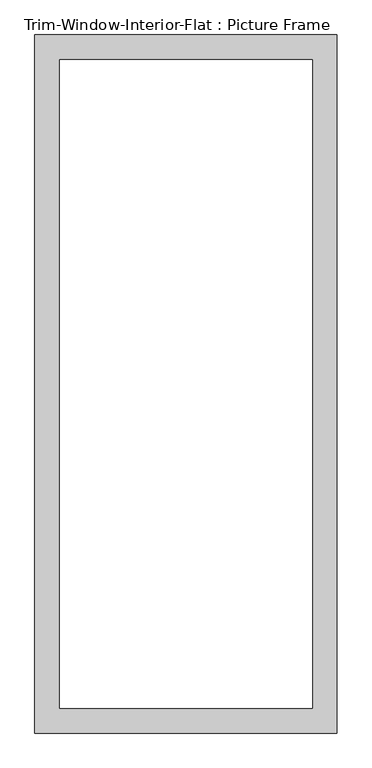
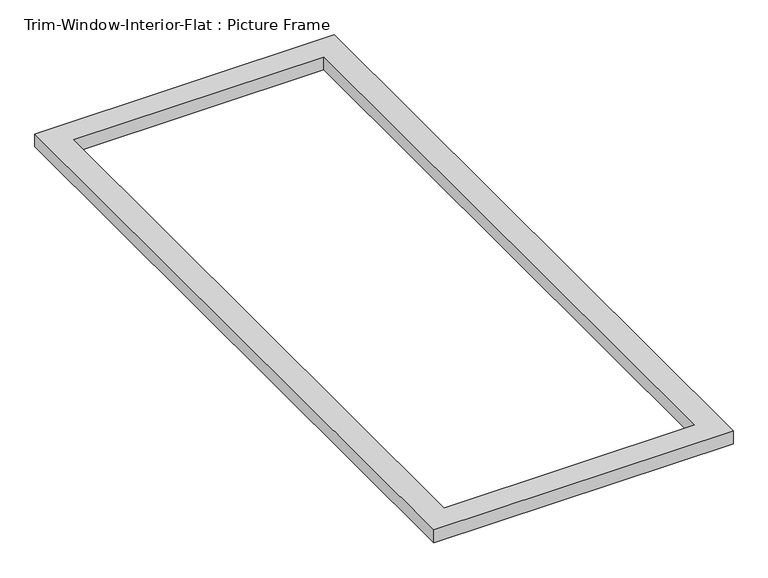
"""IFC4 building model written with IfcOpenShell, lengths in millimetres: proxy geometry, Trim-Window-Interior-Flat : Picture Frame."""

from ifc_helpers import new_model, si_unit, origin, origin_with_axes, place, context, project, spatial, polyline, outline, extrude, source, transform, mapped, element, save


def trim_window_interior_flat_picture_frame_70b72581(model_context):
    return source(origin(), model_context, "Body", "SweptSolid", [
        extrude(outline(polyline([(349.25, -44.45), (-349.25, -44.45), (-349.25, 1568.45), (349.25, 1568.45), (349.25, -44.45)]), holes=[polyline([(292.1, 12.7), (292.1, 1511.3), (-292.1, 1511.3), (-292.1, 12.7), (292.1, 12.7)])]), origin_with_axes(), (0.0, 0.0, 1.0), 31.75),
    ])


if __name__ == "__main__":
    model = new_model("IFC4")
    model_context = context("Model", 3, world=origin())
    ifc_project = project(units=[si_unit("LENGTHUNIT", "METRE", prefix="MILLI")], contexts=[model_context])
    site = spatial("IfcSite", under=ifc_project)
    building = spatial("IfcBuilding", under=site)
    placement = place(None, origin())
    trim_window_interior_flat_picture_frame_shape = trim_window_interior_flat_picture_frame_70b72581(model_context)
    element("IfcBuildingElementProxy", 1, Name="Trim-Window-Interior-Flat : Picture Frame", ObjectType="Trim-Window-Interior-Flat : Picture Frame", at=placement, inside=building, context=model_context, shape_type="MappedRepresentation", body=[
        mapped(trim_window_interior_flat_picture_frame_shape, transform((0.0, 0.0, 0.0), x_axis=(1.0, 0.0, 0.0), y_axis=(0.0, 1.0, 0.0), z_axis=(0.0, 0.0, 1.0))),
    ])
    save(model, "model.ifc")

# Revit data of these elements
# Type "Trim-Window-Interior-Flat : Picture Frame"
#   Trim Thickness_Picture Frame = 0' - 1 1/4"
#   Trim Width = 0' - 2 1/4"
#   Trim Thickness_with Sill = 0' - 0 3/4"
#   Sill Thickness = 0' - 1 1/4"
#   Opening Width [instance default] = 2' - 0"
#   Opening Height [instance default] = 3' - 0"
#   Default Elevation = 4' - 0"
#   Sill = no
#   Picture Frame = yes
#   Trim Material [instance default] = none
# Element 1 (IfcBuildingElementProxy, "Trim-Window-Interior-Flat : Picture Frame")
#   Opening Height = 5' - 0"
#   Trim Material = Wood - Stained
#   Materials on its faces: "Wood - Stained"
# Materials
#   "Wood - Stained": class "Wood", colour RGB 224 178 126, transparency 0, Cost = 0
